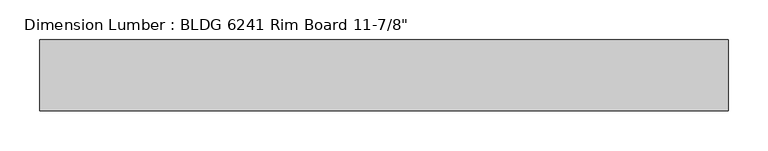
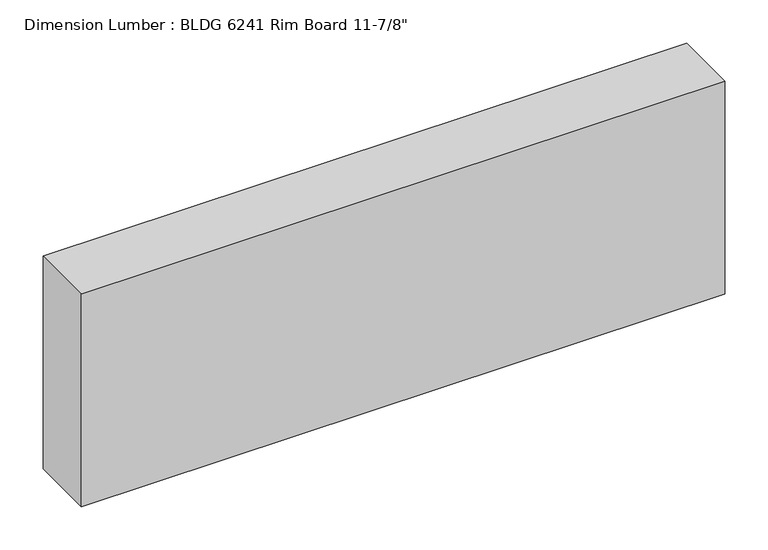
"""IFC4 building model written with IfcOpenShell, lengths in millimetres: beam geometry."""

from ifc_helpers import new_model, si_unit, frame, origin, place, context, project, spatial, polyline, outline, extrude, source, transform, mapped, element, save


def beam_d6a2cfd4(model_context):
    return source(origin(), model_context, "Body", "SweptSolid", [
        extrude(outline(polyline([(431.0522938, 44.45), (431.0522938, -44.45), (-431.0522938, -44.45), (-431.0522938, 44.45), (431.0522938, 44.45)])), frame((0.0, 0.0, -150.8125), z_axis=(0.0, 0.0, 1.0), x_axis=(1.0, 0.0, 0.0)), (0.0, 0.0, 1.0), 301.625),
    ])


if __name__ == "__main__":
    model = new_model("IFC4")
    model_context = context("Model", 3, world=origin())
    ifc_project = project(units=[si_unit("LENGTHUNIT", "METRE", prefix="MILLI")], contexts=[model_context])
    site = spatial("IfcSite", under=ifc_project)
    building = spatial("IfcBuilding", under=site)
    placement = place(None, origin())
    beam_shape = beam_d6a2cfd4(model_context)
    element("IfcBeam", 1, ObjectType="Dimension Lumber : BLDG 6241 Rim Board 11-7/8\"", at=placement, inside=building, context=model_context, shape_type="MappedRepresentation", body=[
        mapped(beam_shape, transform((0.0, 0.0, 0.0), x_axis=(1.0, 0.0, 0.0), y_axis=(0.0, 1.0, 0.0), z_axis=(0.0, 0.0, 1.0))),
    ])
    save(model, "model.ifc")

# Revit data of these elements
# Type "Dimension Lumber : BLDG 6241 Rim Board 11-7/8\""
#   Assembly Code = "B10"
#   A = 0.273472 SF
#   Length [instance default] = 5' - 0"
#   b = 0' - 3 1/2"
#   d = 0' - 11 7/8"
#   Structural Material [instance default] = Softwood, Lumber
# Element 1 (IfcBeam, "Dimension Lumber : BLDG 6241 Rim Board 11-7/8\"")
#   Materials on its faces: "Softwood, Lumber"
# Materials
#   "Softwood, Lumber": class "Wood", colour RGB 223 192 134, transparency 0, Description = "Pinus Echinata", Cost = 0
